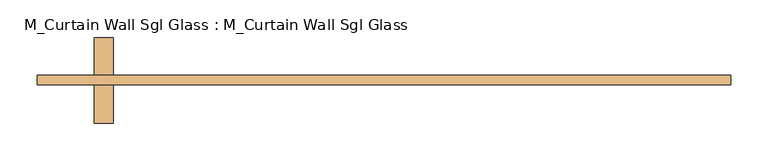
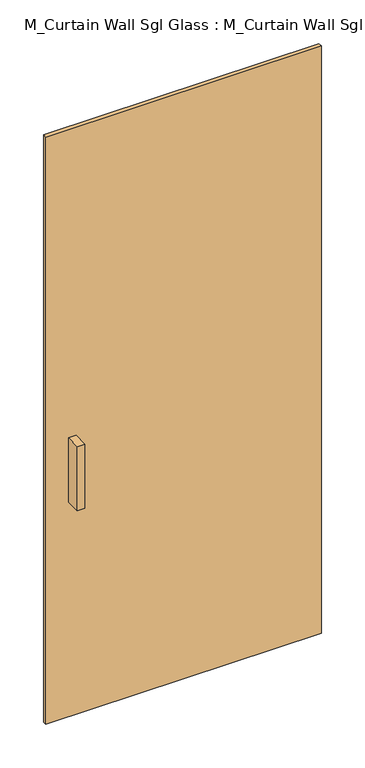
"""IFC4 building model written with IfcOpenShell, lengths in millimetres: door geometry, M_Curtain Wall Sgl Glass : M_Curtain Wall Sgl Glass."""

from ifc_helpers import new_model, si_unit, frame, origin, origin_with_axes, place, context, project, spatial, polyline, outline, extrude, source, transform, mapped, element, save


def m_curtain_wall_sgl_glass_m_curtain_wall_sgl_glass_0d948820(model_context):
    return source(origin(), model_context, "Body", "SweptSolid", [
        extrude(outline(polyline([(-361.3250248, 12.5), (-361.3250248, -38.3), (-386.7250248, -38.3), (-386.7250248, 12.5), (-361.3250248, 12.5)])), frame((0.0, 0.0, 762.0), z_axis=(0.0, 0.0, 1.0), x_axis=(1.0, 0.0, 0.0)), (0.0, 0.0, 1.0), 228.6),
        extrude(outline(polyline([(-386.7250248, -101.8), (-386.7250248, -51.0), (-361.3250248, -51.0), (-361.3250248, -101.8), (-386.7250248, -101.8)])), frame((0.0, 0.0, 762.0), z_axis=(0.0, 0.0, 1.0), x_axis=(1.0, 0.0, 0.0)), (0.0, 0.0, 1.0), 228.6),
        extrude(outline(polyline([(462.9250248, -51.0), (-462.9250248, -51.0), (-462.9250248, -38.3), (462.9250248, -38.3), (462.9250248, -51.0)])), origin_with_axes(), (0.0, 0.0, 1.0), 2085.0),
    ])


if __name__ == "__main__":
    model = new_model("IFC4")
    model_context = context("Model", 3, world=origin())
    ifc_project = project(units=[si_unit("LENGTHUNIT", "METRE", prefix="MILLI")], contexts=[model_context])
    site = spatial("IfcSite", under=ifc_project)
    building = spatial("IfcBuilding", under=site)
    placement = place(None, origin())
    m_curtain_wall_sgl_glass_m_curtain_wall_sgl_glass_shape = m_curtain_wall_sgl_glass_m_curtain_wall_sgl_glass_0d948820(model_context)
    element("IfcDoor", 1, ObjectType="M_Curtain Wall Sgl Glass : M_Curtain Wall Sgl Glass", at=placement, inside=building, context=model_context, shape_type="MappedRepresentation", body=[
        mapped(m_curtain_wall_sgl_glass_m_curtain_wall_sgl_glass_shape, transform((0.0, 0.0, 0.0), x_axis=(1.0, 0.0, 0.0), y_axis=(0.0, 1.0, 0.0), z_axis=(0.0, 0.0, 1.0))),
    ])
    save(model, "model.ifc")

# Revit data of these elements
# Type "M_Curtain Wall Sgl Glass : M_Curtain Wall Sgl Glass"
#   Type Mark = "40"
#   COBie.Type.CreatedBy = "design@eagle.com"
#   COBie.Type.CreatedOn = "2016-09-13T05:47:35"
#   COBie.Type.Name = "Doors_M_Curtain Wall Sgl Glass_M_Curtain Wall Sgl Glass"
#   COBie.Type.Category = "23-30 10 00 : Doors"
#   COBie.Type.Description = ""
#   COBie.Type.Manufacturer = ""
#   COBie.Type.ModelNumber = ""
#   Construction Type Id = "SGL"
#   Analytic Construction = "Large single-glazed windows"
#   COBie.Type.ReplacementCost = 0
#   Visual Light Transmittance = 0.9
#   Solar Heat Gain Coefficient = 0.86
#   Offset = 51 mm
#   Heat Transfer Coefficient (U) = 5.5617 W/(m²·K)
#   COBie.Type = yes
#   Function = 1
#   Glazing Material = Glass
# Element 1 (IfcDoor, "M_Curtain Wall Sgl Glass : M_Curtain Wall Sgl Glass")
#   Materials on its faces: "Aluminum", "Glass"
# Materials
#   "Glass": class "Glass", colour RGB 0 128 192, transparency 0.75, Description = "Soda Lime Glass", Cost = 0
#   "Aluminum": class "Metal", colour RGB 247 247 247, transparency 0, Description = "Aluminum 6061", Cost = 0
